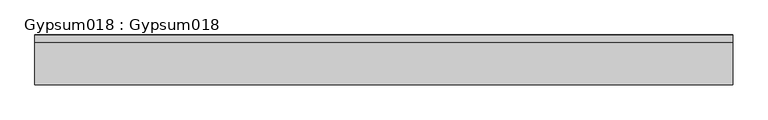
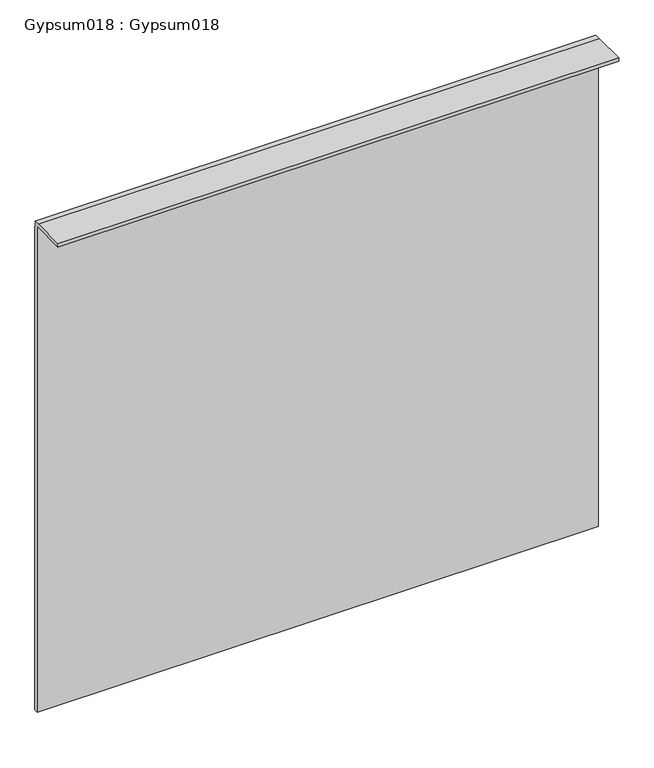
"""IFC4 building model written with IfcOpenShell, lengths in millimetres: proxy geometry, Gypsum018 : Gypsum018."""

from ifc_helpers import new_model, si_unit, frame, origin, place, context, project, spatial, polyline, outline, extrude, source, transform, mapped, element, save


def gypsum018_gypsum018_51115563(model_context):
    return source(origin(), model_context, "Body", "SweptSolid", [
        extrude(outline(polyline([(-4483.5542972, 36582.096), (-4497.8425368, 36582.096), (-4497.8425368, 38414.5015625), (-4625.6960524, 38414.5015625), (-4625.6960524, 38427.7398437), (-4505.9874811, 38427.7398437), (-4505.9874811, 38426.4598437), (-4484.8342972, 38426.4598437), (-4484.8342972, 38405.3066598), (-4483.5542972, 38405.3066598), (-4483.5542972, 36582.096)])), frame((12383.0178845, 0.0, 0.0), z_axis=(1.0, 0.0, 0.0), x_axis=(0.0, 1.0, 0.0)), (0.0, 0.0, 1.0), 2000.0),
    ])


if __name__ == "__main__":
    model = new_model("IFC4")
    model_context = context("Model", 3, world=origin())
    ifc_project = project(units=[si_unit("LENGTHUNIT", "METRE", prefix="MILLI")], contexts=[model_context])
    site = spatial("IfcSite", under=ifc_project)
    building = spatial("IfcBuilding", under=site)
    placement = place(None, origin())
    gypsum018_gypsum018_shape = gypsum018_gypsum018_51115563(model_context)
    element("IfcBuildingElementProxy", 1, Name="Gypsum018 : Gypsum018", ObjectType="Gypsum018 : Gypsum018", at=placement, inside=building, context=model_context, shape_type="MappedRepresentation", body=[
        mapped(gypsum018_gypsum018_shape, transform((0.0, 0.0, 0.0), x_axis=(1.0, 0.0, 0.0), y_axis=(0.0, 1.0, 0.0), z_axis=(0.0, 0.0, 1.0))),
    ])
    save(model, "model.ifc")

# Revit data of these elements
# Type "Gypsum018 : Gypsum018"
#   NameOverride = "Gypsum018"
# Element 1 (IfcBuildingElementProxy, "Gypsum018 : Gypsum018")
#   Materials on its faces: "5/8\"  GYPSUM BOARD"
# Materials
#   "5/8\"  GYPSUM BOARD": class "Unassigned", colour RGB 255 255 255, transparency 0, Cost = 0
